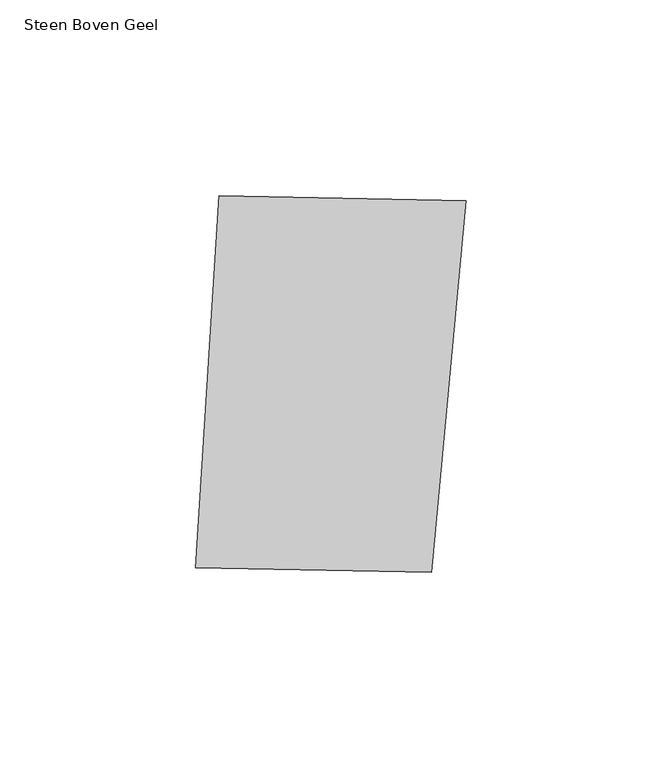
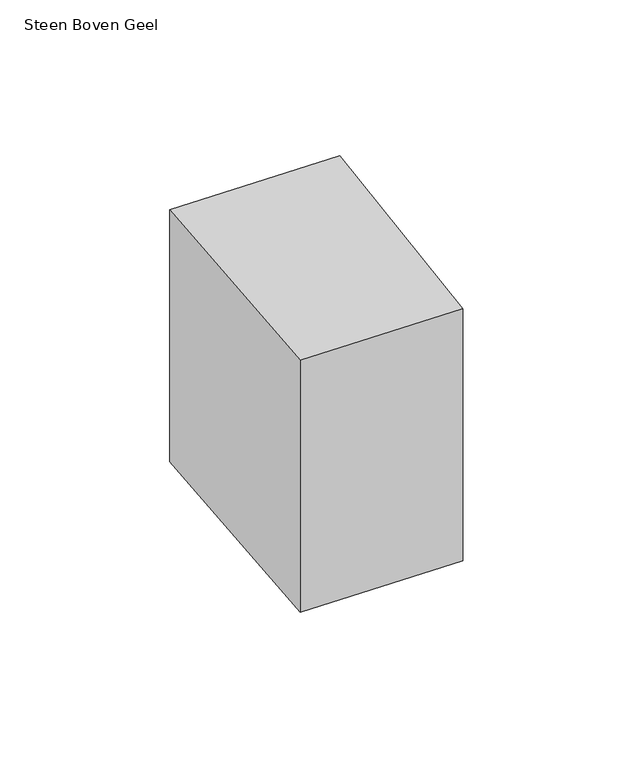
"""IFC4 building model written with IfcOpenShell, lengths in millimetres: proxy geometry, 00_GMA_steen_versie_4 : Steen Boven Geel."""

from ifc_helpers import new_model, si_unit, origin, origin_with_axes, place, context, project, spatial, polyline, outline, extrude, source, transform, mapped, element, save


def steen_boven_geel_de1e0d20(model_context):
    return source(origin(), model_context, "Body", "SweptSolid", [
        extrude(outline(polyline([(105.1638814, 118.6129018), (96.4039791, 23.7504484), (36.1159179, 24.9114518), (42.0985049, 119.8197632), (105.1638814, 118.6129018)])), origin_with_axes(), (0.0, 0.0, 1.0), 100.0),
    ])


if __name__ == "__main__":
    model = new_model("IFC4")
    model_context = context("Model", 3, world=origin())
    ifc_project = project(units=[si_unit("LENGTHUNIT", "METRE", prefix="MILLI")], contexts=[model_context])
    site = spatial("IfcSite", under=ifc_project)
    building = spatial("IfcBuilding", under=site)
    placement = place(None, origin())
    steen_boven_geel_shape = steen_boven_geel_de1e0d20(model_context)
    element("IfcBuildingElementProxy", 1, Name="00_GMA_steen_versie_4 : Steen Boven Geel", ObjectType="00_GMA_steen_versie_4 : Steen Boven Geel", at=placement, inside=building, context=model_context, shape_type="MappedRepresentation", body=[
        mapped(steen_boven_geel_shape, transform((0.0, 0.0, 0.0), x_axis=(1.0, 0.0, 0.0), y_axis=(0.0, 1.0, 0.0), z_axis=(0.0, 0.0, 1.0))),
    ])
    save(model, "model.ifc")

# Revit data of these elements
# Type "00_GMA_steen_versie_4 : Steen Boven Geel"
#   StootVoegHalfBoven [instance default] = 5 mm
#   StootVoegHalf [instance default] = 5 mm
#   StootVoegBreedteOnder = 10 mm
#   StootVoegBreedteBoven = 10 mm
#   Steendikte = 100 mm
#   LintVoegOnderHalf = 5 mm
#   LintVoegOnder = 10 mm
#   LintVoegBovenHalf = 0 mm
#   LintVoegBoven = 0 mm
#   materiaal = 21_steen_geel
#   MateriaalVoeg = none
#   Default Elevation = 0
# Element 1 (IfcBuildingElementProxy, "00_GMA_steen_versie_4 : Steen Boven Geel")
#   Materials on its faces: "21_steen_geel"
# Materials
#   "21_steen_geel": class "Unassigned", colour RGB 202 202 0, transparency 0, Cost = 0
